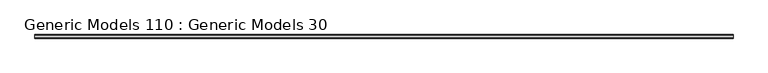
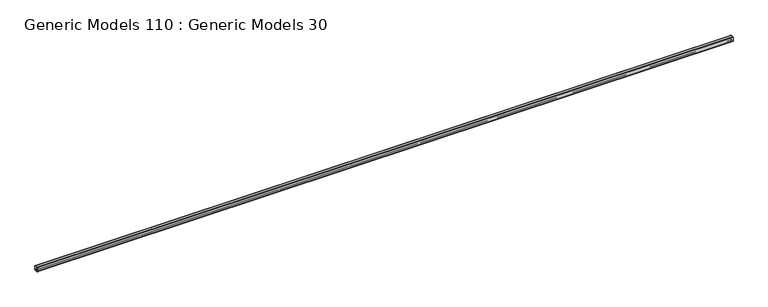
"""IFC4 building model written with IfcOpenShell, lengths in millimetres: proxy geometry, Generic Models 110 : Generic Models 30."""

from ifc_helpers import new_model, si_unit, point, frame, frame_2d, origin, place, context, project, spatial, polyline, circle_curve, trimmed, segment, composite_curve, outline, extrude, source, transform, mapped, element, save


def generic_models_110_generic_models_30_b78b425f(model_context):
    return source(origin(), model_context, "Body", "SweptSolid", [
        extrude(outline(composite_curve([segment(polyline([(41056.1971612, 268943.2516016), (41091.2491612, 268943.2516016)]), True, "CONTINUOUS"), segment(trimmed(circle_curve(frame_2d((41091.2491612, 268936.9016016)), 6.35), [point((41091.2491612, 268943.2516016))], [point((41097.5991612, 268936.9016016))], False, "CARTESIAN"), True, "CONTINUOUS"), segment(polyline([(41097.5991612, 268936.9016016), (41097.5991612, 268888.6416016)]), True, "CONTINUOUS"), segment(trimmed(circle_curve(frame_2d((41091.2491612, 268888.6416016)), 6.35), [point((41097.5991612, 268888.6416016))], [point((41091.2491612, 268882.2916016))], False, "CARTESIAN"), True, "CONTINUOUS"), segment(polyline([(41091.2491612, 268882.2916016), (41085.8404759, 268882.2916016)]), True, "CONTINUOUS"), segment(trimmed(circle_curve(frame_2d((41085.8404759, 268883.8791016)), 1.5875), [point((41085.8404759, 268882.2916016))], [point((41084.2821428, 268883.5761923))], False, "CARTESIAN"), True, "CONTINUOUS"), segment(polyline([(41084.2821428, 268883.5761923), (41082.8566271, 268890.9098347), (41084.3727641, 268890.9098347), (41085.7586863, 268883.7798828), (41091.2491612, 268883.7798828)]), True, "CONTINUOUS"), segment(trimmed(circle_curve(frame_2d((41091.2491612, 268888.6416016)), 4.8617188), [point((41091.2491612, 268883.7798828))], [point((41096.1108799, 268888.6416016))], True, "CARTESIAN"), True, "CONTINUOUS"), segment(polyline([(41096.1108799, 268888.6416016), (41096.1108799, 268936.9016016)]), True, "CONTINUOUS"), segment(trimmed(circle_curve(frame_2d((41091.2491612, 268936.9016016)), 4.8617188), [point((41096.1108799, 268936.9016016))], [point((41091.2491612, 268941.7633203))], True, "CARTESIAN"), True, "CONTINUOUS"), segment(polyline([(41091.2491612, 268941.7633203), (41056.1971612, 268941.7633203)]), True, "CONTINUOUS"), segment(trimmed(circle_curve(frame_2d((41056.1971612, 268936.9016016)), 4.8617188), [point((41056.1971612, 268941.7633203))], [point((41051.3354424, 268936.9016016))], True, "CARTESIAN"), True, "CONTINUOUS"), segment(polyline([(41051.3354424, 268936.9016016), (41051.3354424, 268888.6416016)]), True, "CONTINUOUS"), segment(trimmed(circle_curve(frame_2d((41056.1971612, 268888.6416016)), 4.8617188), [point((41051.3354424, 268888.6416016))], [point((41056.1971612, 268883.7798828))], True, "CARTESIAN"), True, "CONTINUOUS"), segment(polyline([(41056.1971612, 268883.7798828), (41061.6876361, 268883.7798828), (41063.0735583, 268890.9098347), (41064.5896953, 268890.9098347), (41063.1641796, 268883.5761923)]), True, "CONTINUOUS"), segment(trimmed(circle_curve(frame_2d((41061.6058465, 268883.8791016)), 1.5875), [point((41063.1641796, 268883.5761923))], [point((41061.6058465, 268882.2916016))], False, "CARTESIAN"), True, "CONTINUOUS"), segment(polyline([(41061.6058465, 268882.2916016), (41056.1971612, 268882.2916016)]), True, "CONTINUOUS"), segment(trimmed(circle_curve(frame_2d((41056.1971612, 268888.6416016)), 6.35), [point((41056.1971612, 268882.2916016))], [point((41049.8471612, 268888.6416016))], False, "CARTESIAN"), True, "CONTINUOUS"), segment(polyline([(41049.8471612, 268888.6416016), (41049.8471612, 268936.9016016)]), True, "CONTINUOUS"), segment(trimmed(circle_curve(frame_2d((41056.1971612, 268936.9016016)), 6.35), [point((41049.8471612, 268936.9016016))], [point((41056.1971612, 268943.2516016))], False, "CARTESIAN"), True, "CONTINUOUS")], self_intersect=False)), frame((26437.0233878, 0.0, 0.0), z_axis=(1.0, 0.0, 0.0), x_axis=(0.0, 1.0, 0.0)), (0.0, 0.0, 1.0), 9065.0343422),
    ])


if __name__ == "__main__":
    model = new_model("IFC4")
    model_context = context("Model", 3, world=origin())
    ifc_project = project(units=[si_unit("LENGTHUNIT", "METRE", prefix="MILLI")], contexts=[model_context])
    site = spatial("IfcSite", under=ifc_project)
    building = spatial("IfcBuilding", under=site)
    placement = place(None, origin())
    generic_models_110_generic_models_30_shape = generic_models_110_generic_models_30_b78b425f(model_context)
    element("IfcBuildingElementProxy", 1, Name="Generic Models 110 : Generic Models 30", ObjectType="Generic Models 110 : Generic Models 30", at=placement, inside=building, context=model_context, shape_type="MappedRepresentation", body=[
        mapped(generic_models_110_generic_models_30_shape, transform((0.0, 0.0, 0.0), x_axis=(1.0, 0.0, 0.0), y_axis=(0.0, 1.0, 0.0), z_axis=(0.0, 0.0, 1.0))),
    ])
    save(model, "model.ifc")

# Revit data of these elements
# Element 1 (IfcBuildingElementProxy, "Generic Models 110 : Generic Models 30")
#   Materials on its faces: "GALV. BOX RAIL"
# Materials
#   "GALV. BOX RAIL": class "Generic", colour RGB 212 212 212, transparency 0, Cost = 0
